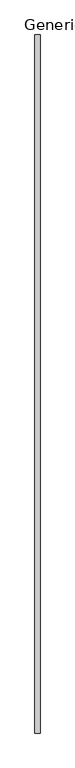
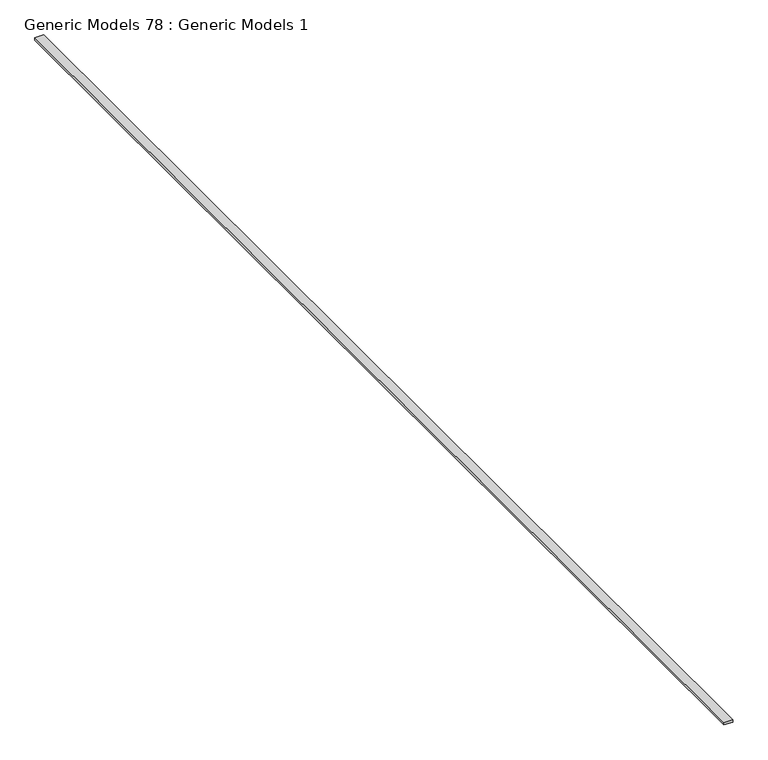
"""IFC4 building model written with IfcOpenShell, lengths in millimetres: proxy geometry, Generic Models 78 : Generic Models 1."""

from ifc_helpers import new_model, si_unit, frame, origin, place, context, project, spatial, polyline, outline, extrude, source, transform, mapped, element, save


def generic_models_78_generic_models_1_067f4f74(model_context):
    return source(origin(), model_context, "Body", "SweptSolid", [
        extrude(outline(polyline([(8188.1513704, 11981.8769662), (8327.8513704, 11981.8769662), (8327.8513704, -7068.1230338), (8188.1513704, -7068.1230338), (8188.1513704, 11981.8769662)])), frame((0.0, 0.0, 127028.2735933), z_axis=(0.0, 0.0, 1.0), x_axis=(1.0, 0.0, 0.0)), (0.0, 0.0, 1.0), 38.1),
    ])


if __name__ == "__main__":
    model = new_model("IFC4")
    model_context = context("Model", 3, world=origin())
    ifc_project = project(units=[si_unit("LENGTHUNIT", "METRE", prefix="MILLI")], contexts=[model_context])
    site = spatial("IfcSite", under=ifc_project)
    building = spatial("IfcBuilding", under=site)
    placement = place(None, origin())
    generic_models_78_generic_models_1_shape = generic_models_78_generic_models_1_067f4f74(model_context)
    element("IfcBuildingElementProxy", 1, Name="Generic Models 78 : Generic Models 1", ObjectType="Generic Models 78 : Generic Models 1", at=placement, inside=building, context=model_context, shape_type="MappedRepresentation", body=[
        mapped(generic_models_78_generic_models_1_shape, transform((0.0, 0.0, 0.0), x_axis=(1.0, 0.0, 0.0), y_axis=(0.0, 1.0, 0.0), z_axis=(0.0, 0.0, 1.0))),
    ])
    save(model, "model.ifc")

# Revit data of these elements
# Element 1 (IfcBuildingElementProxy, "Generic Models 78 : Generic Models 1")
#   Materials on its faces: "_2X BLOCKING AS REQUIRED"
# Materials
#   "_2X BLOCKING AS REQUIRED": class "Generic", colour RGB 177 130 114, transparency 0, Cost = 0
